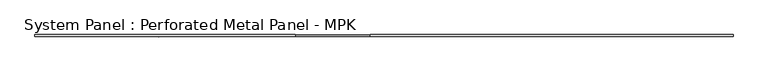
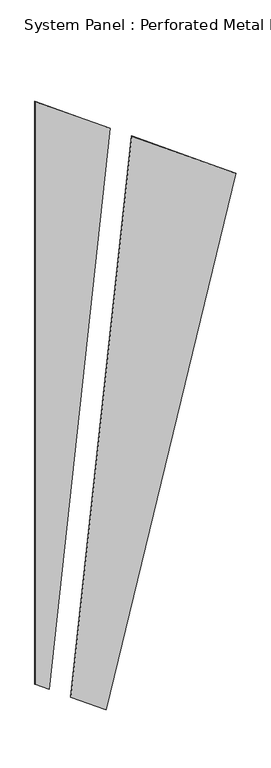
"""IFC4 building model written with IfcOpenShell, lengths in millimetres: plate geometry, System Panel : Perforated Metal Panel - MPK."""

from ifc_helpers import new_model, si_unit, frame, origin, place, context, project, spatial, polyline, outline, extrude, source, transform, mapped, element, save


def system_panel_perforated_metal_panel_mpk_e5f3f07d(model_context):
    return source(origin(), model_context, "Body", "SweptSolid", [
        extrude(outline(polyline([(990.4856918, -2509.8848507), (0.0, -1146.0672019), (20185.1046475, 3890.7832032), (23120.5989905, -151.152007), (990.4856918, -2509.8848507)])), frame((0.0, 0.0, 0.0), z_axis=(0.0, 1.0, 0.0), x_axis=(0.0, 0.0, 1.0)), (0.0, 0.0, 1.0), 20.0),
        extrude(outline(polyline([(1993.3764091, -3890.7832032), (1600.3887358, -3349.6713738), (23730.5020345, -990.9385302), (25836.5421342, -3890.7832032), (1993.3764091, -3890.7832032)])), frame((0.0, 0.0, 0.0), z_axis=(0.0, 1.0, 0.0), x_axis=(0.0, 0.0, 1.0)), (0.0, 0.0, 1.0), 20.0),
    ])


if __name__ == "__main__":
    model = new_model("IFC4")
    model_context = context("Model", 3, world=origin())
    ifc_project = project(units=[si_unit("LENGTHUNIT", "METRE", prefix="MILLI")], contexts=[model_context])
    site = spatial("IfcSite", under=ifc_project)
    building = spatial("IfcBuilding", under=site)
    placement = place(None, origin())
    system_panel_perforated_metal_panel_mpk_shape = system_panel_perforated_metal_panel_mpk_e5f3f07d(model_context)
    element("IfcPlate", 1, ObjectType="System Panel : Perforated Metal Panel - MPK", at=placement, inside=building, context=model_context, shape_type="MappedRepresentation", body=[
        mapped(system_panel_perforated_metal_panel_mpk_shape, transform((0.0, 0.0, 0.0), x_axis=(1.0, 0.0, 0.0), y_axis=(0.0, 1.0, 0.0), z_axis=(0.0, 0.0, 1.0))),
    ])
    save(model, "model.ifc")

# Revit data of these elements
# Element 1 (IfcPlate, "System Panel : Perforated Metal Panel - MPK")
#   Materials on its faces: "Perforated  Metal Panels - MPK"
# Materials
#   "Perforated  Metal Panels - MPK": class "Miscellaneous", colour RGB 127 127 127, transparency 0
